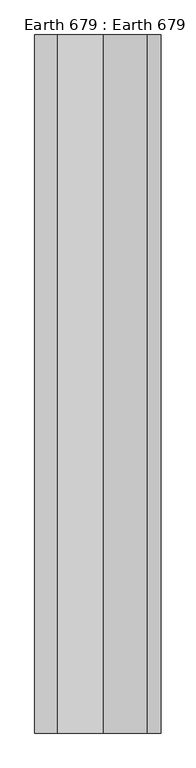
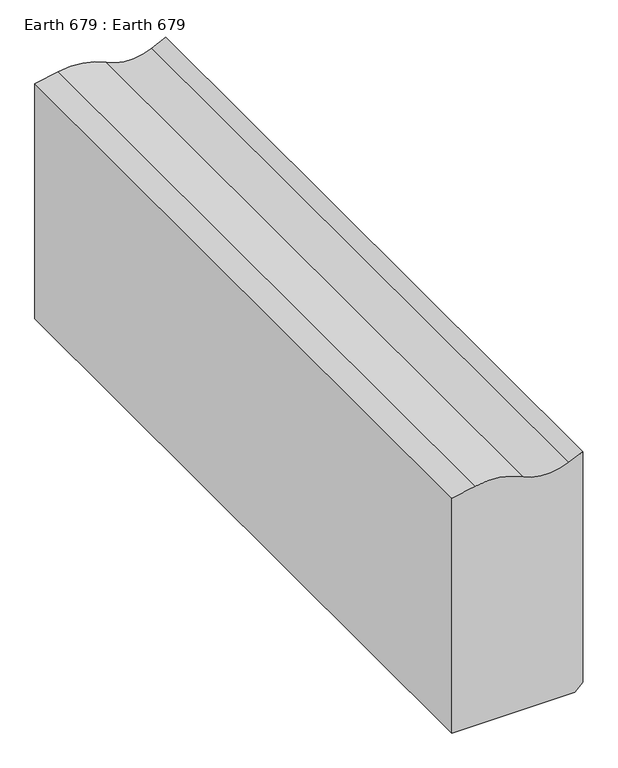
"""IFC4 building model written with IfcOpenShell, lengths in millimetres: proxy geometry, Earth 679 : Earth 679."""

from ifc_helpers import new_model, si_unit, point, frame, frame_2d, origin, place, context, project, spatial, polyline, circle_curve, trimmed, segment, composite_curve, outline, extrude, source, transform, mapped, element, save


def earth_679_earth_679_1ffde3c4(model_context):
    return source(origin(), model_context, "Body", "SweptSolid", [
        extrude(outline(composite_curve([segment(polyline([(32620.9902343, -10057.5706312), (32620.9902343, -9717.2148439), (32643.1028304, -9695.1022478), (33318.0501956, -9695.1022478), (33300.0908366, -9733.8927957)]), True, "CONTINUOUS"), segment(trimmed(circle_curve(frame_2d((33431.3167137, -9794.6481283)), 144.607888), [point((33300.0908366, -9733.8927957))], [point((33302.6181918, -9860.5884932))], True, "CARTESIAN"), True, "CONTINUOUS"), segment(trimmed(circle_curve(frame_2d((33120.1913863, -9954.0572443)), 204.9779178), [point((33302.6181918, -9860.5884932))], [point((33321.4784396, -9992.7802216))], False, "CARTESIAN"), True, "CONTINUOUS"), segment(polyline([(33321.4784396, -9992.7802216), (33309.014262, -10057.5706312), (32620.9902343, -10057.5706312)]), True, "CONTINUOUS")], self_intersect=False)), frame((0.0, 7982.1531721, 0.0), z_axis=(0.0, 1.0, 0.0), x_axis=(0.0, 0.0, 1.0)), (0.0, 0.0, 1.0), 2000.0),
    ])


if __name__ == "__main__":
    model = new_model("IFC4")
    model_context = context("Model", 3, world=origin())
    ifc_project = project(units=[si_unit("LENGTHUNIT", "METRE", prefix="MILLI")], contexts=[model_context])
    site = spatial("IfcSite", under=ifc_project)
    building = spatial("IfcBuilding", under=site)
    placement = place(None, origin())
    earth_679_earth_679_shape = earth_679_earth_679_1ffde3c4(model_context)
    element("IfcBuildingElementProxy", 1, Name="Earth 679 : Earth 679", ObjectType="Earth 679 : Earth 679", at=placement, inside=building, context=model_context, shape_type="MappedRepresentation", body=[
        mapped(earth_679_earth_679_shape, transform((0.0, 0.0, 0.0), x_axis=(1.0, 0.0, 0.0), y_axis=(0.0, 1.0, 0.0), z_axis=(0.0, 0.0, 1.0))),
    ])
    save(model, "model.ifc")

# Revit data of these elements
# Type "Earth 679 : Earth 679"
#   NameOverride = "Earth"
# Element 1 (IfcBuildingElementProxy, "Earth 679 : Earth 679")
#   Materials on its faces: "GROUND SOIL"
# Materials
#   "GROUND SOIL": class "Unassigned", colour RGB 170 124 75, transparency 0, Cost = 0
